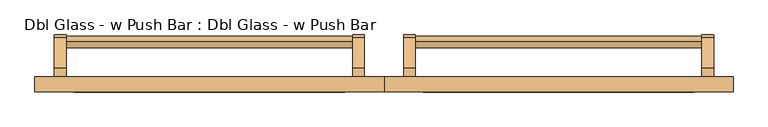
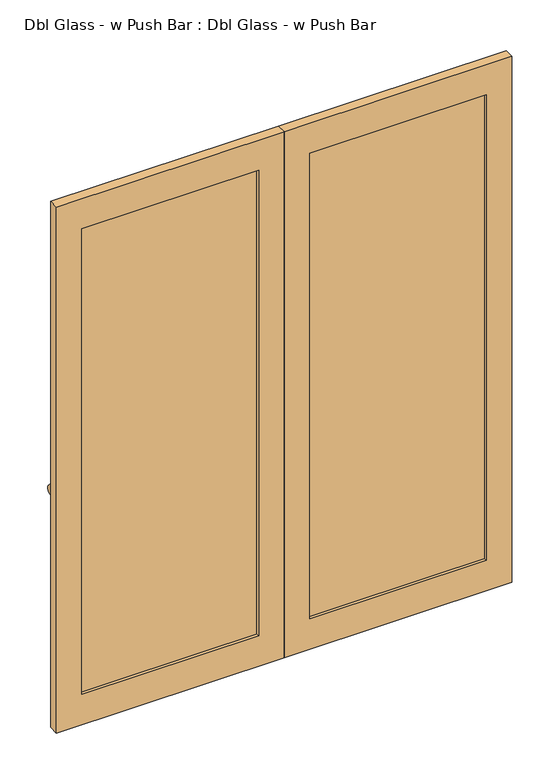
"""IFC4 building model written with IfcOpenShell, lengths in millimetres: door geometry, Dbl Glass - w Push Bar : Dbl Glass - w Push Bar."""

from ifc_helpers import new_model, si_unit, point, frame, frame_2d, origin, place, context, project, spatial, polyline, circle_curve, trimmed, segment, composite_curve, outline, extrude, source, transform, mapped, element, save


def dbl_glass_w_push_bar_dbl_glass_w_push_bar_f1c4d891(model_context):
    return source(origin(), model_context, "Body", "SweptSolid", [
        extrude(outline(composite_curve([segment(trimmed(circle_curve(frame_2d((65.0203019, 909.5721086)), 15.0), [point((65.0203019, 924.5721086))], [point((65.0203019, 894.5721086))], False, "CARTESIAN"), True, "CONTINUOUS"), segment(trimmed(circle_curve(frame_2d((65.0203019, 909.5721086)), 15.0), [point((65.0203019, 894.5721086))], [point((65.0203019, 924.5721086))], False, "CARTESIAN"), True, "CONTINUOUS")], self_intersect=False)), frame((80.0, 0.0, 0.0), z_axis=(1.0, 0.0, 0.0), x_axis=(0.0, 1.0, 0.0)), (0.0, 0.0, 1.0), 731.0),
        extrude(outline(composite_curve([segment(polyline([(-0.1563269, 1000.0), (77.6459332, 922.19774)]), True, "CONTINUOUS"), segment(trimmed(circle_curve(frame_2d((65.0203019, 909.5721086)), 17.8553391), [point((77.6459332, 922.19774))], [point((52.3946705, 896.9464773))], False, "CARTESIAN"), True, "CONTINUOUS"), segment(polyline([(52.3946705, 896.9464773), (14.3411478, 935.0), (-24.035259, 935.0), (-24.035259, 1000.0), (-0.1563269, 1000.0)]), True, "CONTINUOUS")], self_intersect=False)), frame((811.0, 0.0, 0.0), z_axis=(1.0, 0.0, 0.0), x_axis=(0.0, 1.0, 0.0)), (0.0, 0.0, 1.0), 30.0),
        extrude(outline(composite_curve([segment(polyline([(-0.1563269, 1000.0), (77.6459332, 922.19774)]), True, "CONTINUOUS"), segment(trimmed(circle_curve(frame_2d((65.0203019, 909.5721086)), 17.8553391), [point((77.6459332, 922.19774))], [point((52.3946705, 896.9464773))], False, "CARTESIAN"), True, "CONTINUOUS"), segment(polyline([(52.3946705, 896.9464773), (14.3411478, 935.0), (-24.035259, 935.0), (-24.035259, 1000.0), (-0.1563269, 1000.0)]), True, "CONTINUOUS")], self_intersect=False)), frame((50.0, 0.0, 0.0), z_axis=(1.0, 0.0, 0.0), x_axis=(0.0, 1.0, 0.0)), (0.0, 0.0, 1.0), 30.0),
        extrude(outline(composite_curve([segment(trimmed(circle_curve(frame_2d((65.0203019, 909.5721086)), 15.0), [point((65.0203019, 924.5721086))], [point((65.0203019, 894.5721086))], False, "CARTESIAN"), True, "CONTINUOUS"), segment(trimmed(circle_curve(frame_2d((65.0203019, 909.5721086)), 15.0), [point((65.0203019, 894.5721086))], [point((65.0203019, 924.5721086))], False, "CARTESIAN"), True, "CONTINUOUS")], self_intersect=False)), frame((-811.0, 0.0, 0.0), z_axis=(1.0, 0.0, 0.0), x_axis=(0.0, 1.0, 0.0)), (0.0, 0.0, 1.0), 731.0),
        extrude(outline(composite_curve([segment(polyline([(-0.1563269, 1000.0), (77.6459332, 922.19774)]), True, "CONTINUOUS"), segment(trimmed(circle_curve(frame_2d((65.0203019, 909.5721086)), 17.8553391), [point((77.6459332, 922.19774))], [point((52.3946705, 896.9464773))], False, "CARTESIAN"), True, "CONTINUOUS"), segment(polyline([(52.3946705, 896.9464773), (14.3411478, 935.0), (-24.035259, 935.0), (-24.035259, 1000.0), (-0.1563269, 1000.0)]), True, "CONTINUOUS")], self_intersect=False)), frame((-80.0, 0.0, 0.0), z_axis=(1.0, 0.0, 0.0), x_axis=(0.0, 1.0, 0.0)), (0.0, 0.0, 1.0), 30.0),
        extrude(outline(composite_curve([segment(polyline([(-0.1563269, 1000.0), (77.6459332, 922.19774)]), True, "CONTINUOUS"), segment(trimmed(circle_curve(frame_2d((65.0203019, 909.5721086)), 17.8553391), [point((77.6459332, 922.19774))], [point((52.3946705, 896.9464773))], False, "CARTESIAN"), True, "CONTINUOUS"), segment(polyline([(52.3946705, 896.9464773), (14.3411478, 935.0), (-24.035259, 935.0), (-24.035259, 1000.0), (-0.1563269, 1000.0)]), True, "CONTINUOUS")], self_intersect=False)), frame((-841.0, 0.0, 0.0), z_axis=(1.0, 0.0, 0.0), x_axis=(0.0, 1.0, 0.0)), (0.0, 0.0, 1.0), 30.0),
        extrude(outline(polyline([(2175.0, -891.0), (0.0, -891.0), (0.0, 0.0), (2175.0, 0.0), (2175.0, -891.0)]), holes=[polyline([(2050.0, -791.0), (2050.0, -100.0), (125.0, -100.0), (125.0, -791.0), (2050.0, -791.0)])]), frame((0.0, -62.5788556, 0.0), z_axis=(0.0, 1.0, 0.0), x_axis=(0.0, 0.0, 1.0)), (0.0, 0.0, 1.0), 38.5435966),
        extrude(outline(polyline([(2175.0, 0.0), (0.0, 0.0), (0.0, 891.0), (2175.0, 891.0), (2175.0, 0.0)]), holes=[polyline([(2050.0, 100.0), (2050.0, 791.0), (125.0, 791.0), (125.0, 100.0), (2050.0, 100.0)])]), frame((0.0, -62.5788556, 0.0), z_axis=(0.0, 1.0, 0.0), x_axis=(0.0, 0.0, 1.0)), (0.0, 0.0, 1.0), 38.5435966),
        extrude(outline(polyline([(-100.0, -38.0), (-100.0, -50.0), (-791.0, -50.0), (-791.0, -38.0), (-100.0, -38.0)])), frame((0.0, 0.0, 125.0), z_axis=(0.0, 0.0, 1.0), x_axis=(1.0, 0.0, 0.0)), (0.0, 0.0, 1.0), 1925.0),
        extrude(outline(polyline([(791.0, -38.0), (791.0, -50.0), (100.0, -50.0), (100.0, -38.0), (791.0, -38.0)])), frame((0.0, 0.0, 125.0), z_axis=(0.0, 0.0, 1.0), x_axis=(1.0, 0.0, 0.0)), (0.0, 0.0, 1.0), 1925.0),
    ])


if __name__ == "__main__":
    model = new_model("IFC4")
    model_context = context("Model", 3, world=origin())
    ifc_project = project(units=[si_unit("LENGTHUNIT", "METRE", prefix="MILLI")], contexts=[model_context])
    site = spatial("IfcSite", under=ifc_project)
    building = spatial("IfcBuilding", under=site)
    placement = place(None, origin())
    dbl_glass_w_push_bar_dbl_glass_w_push_bar_shape = dbl_glass_w_push_bar_dbl_glass_w_push_bar_f1c4d891(model_context)
    element("IfcDoor", 1, ObjectType="Dbl Glass - w Push Bar : Dbl Glass - w Push Bar", at=placement, inside=building, context=model_context, shape_type="MappedRepresentation", body=[
        mapped(dbl_glass_w_push_bar_dbl_glass_w_push_bar_shape, transform((0.0, 0.0, 0.0), x_axis=(1.0, 0.0, 0.0), y_axis=(0.0, 1.0, 0.0), z_axis=(0.0, 0.0, 1.0))),
    ])
    save(model, "model.ifc")

# Revit data of these elements
# Type "Dbl Glass - w Push Bar : Dbl Glass - w Push Bar"
#   Description = "Curtain Wall Door"
#   Type Mark = "55"
#   Construction Type Id = "GSP4R"
#   Analytic Construction = "1/8 in Pilkington single glazing"
#   Visual Light Transmittance = 0.9
#   TopRail = 125 mm
#   Solar Heat Gain Coefficient = 0.78
#   Offset = 50 mm
#   MuntinRail = 100 mm
#   LockRail = 100 mm
#   Heat Transfer Coefficient (U) = 3.6886 W/(m²·K)
#   Handle Z Distance = 1000 mm
#   Handle X Offset = 65 mm
#   Glass Thickness = 12 mm
#   BottomRail = 125 mm
#   Define Thermal Properties by = 1
#   Material Ironmongery = Metal - Aluminum
#   Material Door = Metal - Aluminum
#   Material Glass = Glass
#   Function = (empty or 0)
# Element 1 (IfcDoor, "Dbl Glass - w Push Bar : Dbl Glass - w Push Bar")
#   Materials on its faces: "Metal - Aluminum", "Glass"
# Materials
#   "Metal - Aluminum": class "Metal", colour RGB 247 247 247, transparency 0
#   "Glass": class "Glass", colour RGB 0 128 192, transparency 0.9, Description = "Soda Lime Glass", Cost = 0
